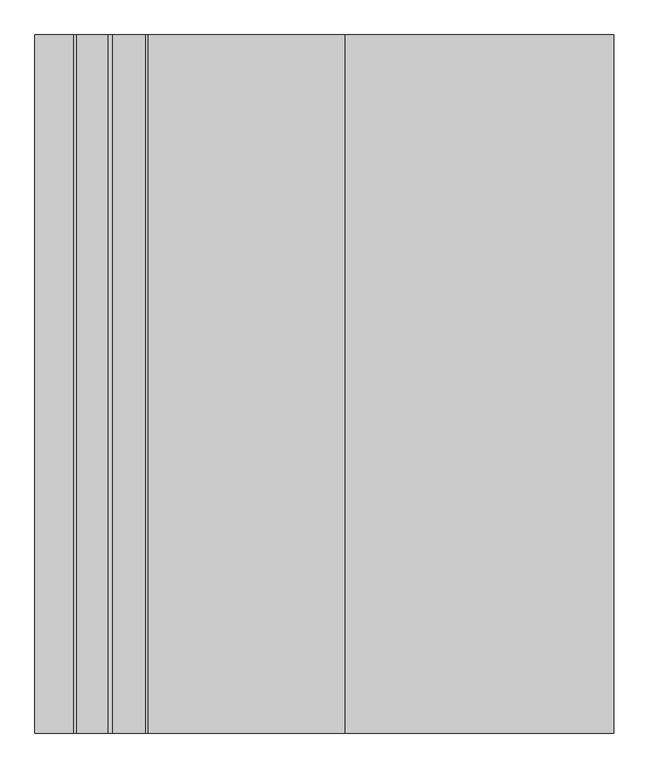
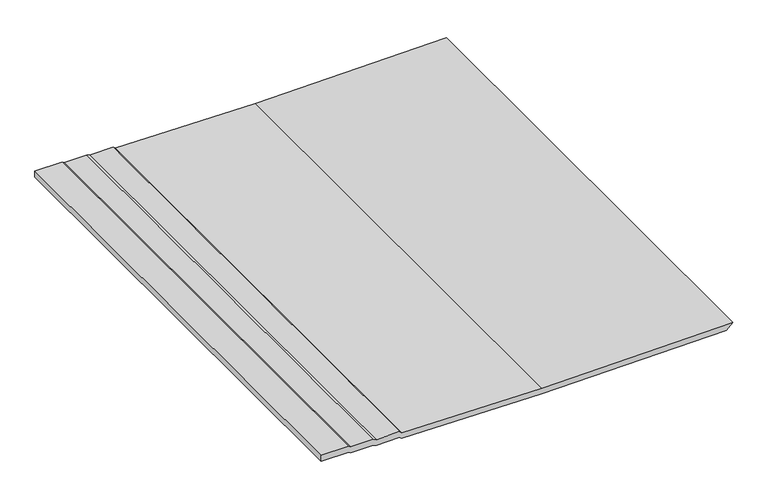
"""IFC4 building model written with IfcOpenShell, lengths in millimetres: proxy geometry, GRAVEL BALLAST002 1:GRAVEL BALLAST002 15468:299766 : GRAVEL BALLAST002 1:GRAVEL BALLAST002 15468:299766."""

from ifc_helpers import new_model, si_unit, frame, origin, place, context, project, spatial, polyline, outline, extrude, source, transform, mapped, element, save


def generic_models_ffe3ee17(model_context):
    return source(origin(), model_context, "Body", "SweptSolid", [
        extrude(outline(polyline([(40274.2359464, 1995.1433186), (40274.2359464, 2104.6428303), (40269.9546964, 2113.3532795), (40269.9546964, 2203.9401936), (40264.2272344, 2216.7848329), (40265.8726651, 2310.7365803), (40258.4625089, 2319.0100178), (40250.2437589, 2882.0804523), (40261.546875, 3627.5723404), (40286.2851563, 3653.5460953), (40274.9820402, 2882.0804523), (40283.2007902, 2319.0100178), (40290.6109464, 2310.7365803), (40288.9655157, 2216.7848329), (40294.6929777, 2203.9401936), (40294.6929777, 2113.3532795), (40298.9742277, 2104.6428303), (40298.9742277, 1995.1433186), (40274.2359464, 1995.1433186)])), frame((0.0, -774.3081162, 0.0), z_axis=(0.0, 1.0, 0.0), x_axis=(0.0, 0.0, 1.0)), (0.0, 0.0, 1.0), 2000.0),
    ])


if __name__ == "__main__":
    model = new_model("IFC4")
    model_context = context("Model", 3, world=origin())
    ifc_project = project(units=[si_unit("LENGTHUNIT", "METRE", prefix="MILLI")], contexts=[model_context])
    site = spatial("IfcSite", under=ifc_project)
    building = spatial("IfcBuilding", under=site)
    placement = place(None, origin())
    generic_models_shape = generic_models_ffe3ee17(model_context)
    element("IfcBuildingElementProxy", 1, Name="GRAVEL BALLAST002 1:GRAVEL BALLAST002 15468:299766 : GRAVEL BALLAST002 1:GRAVEL BALLAST002 15468:299766", ObjectType="GRAVEL BALLAST002 1:GRAVEL BALLAST002 15468:299766 : GRAVEL BALLAST002 1:GRAVEL BALLAST002 15468:299766", at=placement, inside=building, context=model_context, shape_type="MappedRepresentation", body=[
        mapped(generic_models_shape, transform((0.0, 0.0, 0.0), x_axis=(1.0, 0.0, 0.0), y_axis=(0.0, 1.0, 0.0), z_axis=(0.0, 0.0, 1.0))),
    ])
    save(model, "model.ifc")

# Revit data of these elements
# Type "GRAVEL BALLAST002 1:GRAVEL BALLAST002 15468:299766 : GRAVEL BALLAST002 1:GRAVEL BALLAST002 15468:299766"
#   NameOverride = "GRAVEL BALLAST002 1:GRAVEL BALLAST002 15468:299766"
#   ObjectTypeOverride = "GRAVEL BALLAST002 1:GRAVEL BALLAST002 15468"
#   Reference = "GRAVEL BALLAST002 15468"
#   Category = "Generic Models"
#   Tag = "299766"
# Element 1 (IfcBuildingElementProxy, "GRAVEL BALLAST002 1:GRAVEL BALLAST002 15468:299766 : GRAVEL BALLAST002 1:GRAVEL BALLAST002 15468:299766")
#   Materials on its faces: "GRAVEL BALLAST"
# Materials
#   "GRAVEL BALLAST": class "Unassigned", colour RGB 128 128 128, transparency 0, Cost = 0
